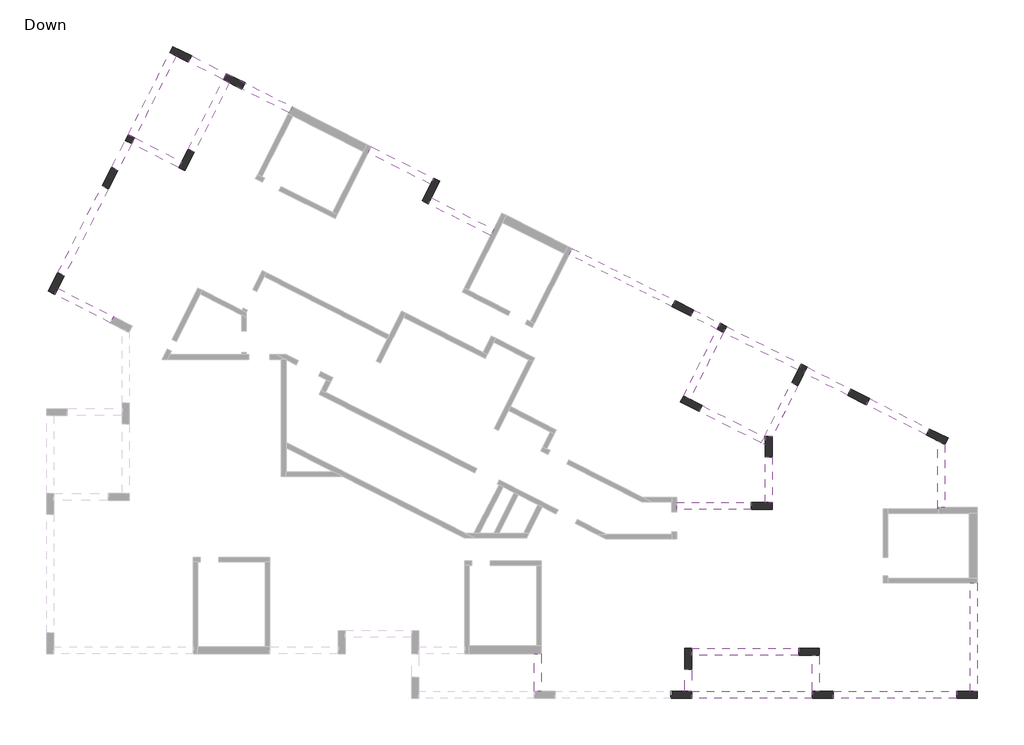
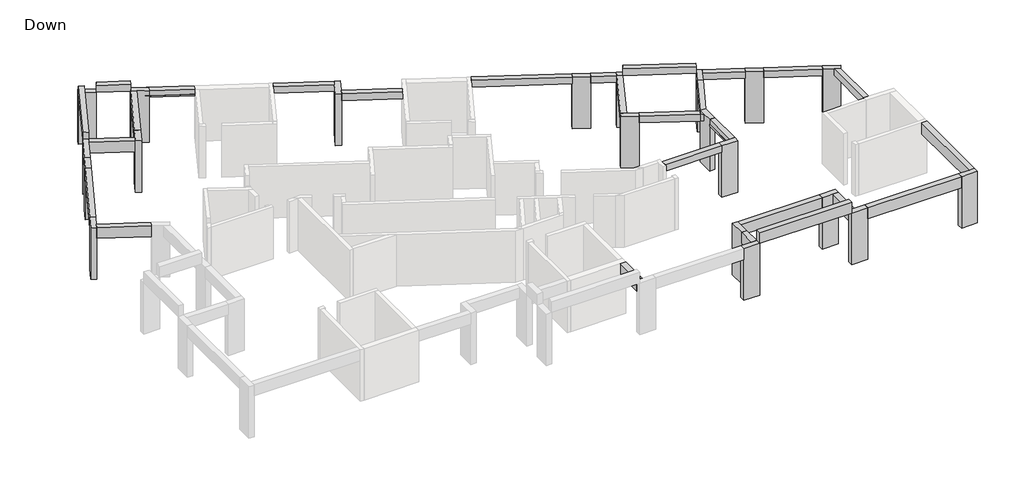
# One storey, part 3 of 3: 28 beams, 20 columns.
"""IFC4 building model written with IfcOpenShell, lengths in millimetres."""

import ifcopenshell
import ifcopenshell.guid

model = None  # the IFC model being written
_history = None  # IfcOwnerHistory: only IFC2X3 demands one
_inside = {}  # id of a spatial element -> (the spatial element, [elements in it])
_under = {}  # id of a project, library or spatial element -> (it, [spatial elements below it])
_declared = {}  # id of a project -> (the project, [libraries it declares])
_typed = {}  # id of a type object -> (the type object, [elements of that type])
_made_of = {}  # id of a material, layer set ... -> (it, [elements and type objects made of it])


def new_model(schema):
    """Start an empty IFC model of exactly this schema.

    Asked for "IFC4X3", IfcOpenShell would pick the latest addendum, in which some entities
    have other attributes; the version numbers below select the first issue.
    IFC2X3 requires an IfcOwnerHistory on every rooted entity: one is made here for all.
    """
    global model, _history
    if schema == "IFC4X3":
        model = ifcopenshell.file(schema_version=(4, 3, 0, 0))
    else:
        model = ifcopenshell.file(schema=schema)
    _inside.clear()
    _under.clear()
    _declared.clear()
    _typed.clear()
    _made_of.clear()
    _history = None
    if model.schema == "IFC2X3":
        org = make("IfcOrganization", Name="unknown")
        user = make(
            "IfcPersonAndOrganization",
            ThePerson=make("IfcPerson", FamilyName="unknown"),
            TheOrganization=org,
        )
        app = make(
            "IfcApplication",
            ApplicationDeveloper=org,
            Version="unknown",
            ApplicationFullName="unknown",
            ApplicationIdentifier="unknown",
        )
        _history = make(
            "IfcOwnerHistory",
            OwningUser=user,
            OwningApplication=app,
            ChangeAction="ADDED",
            CreationDate=0,
        )
    return model


def make(cls, **values):
    """One entity of the class cls with the attributes given. An attribute that is None is left unset."""
    return model.create_entity(
        cls, **{name: value for name, value in values.items() if value is not None}
    )


def rooted(cls, **values):
    """An entity with a GlobalId (a new one), such as an element, a storey or a relation."""
    return make(cls, GlobalId=ifcopenshell.guid.new(), OwnerHistory=_history, **values)


def si_unit(unit_type, name, prefix=None):
    """IfcSIUnit, for example si_unit("LENGTHUNIT", "METRE", prefix="MILLI")."""
    return make("IfcSIUnit", UnitType=unit_type, Prefix=prefix, Name=name)


def assignment(units):
    """IfcUnitAssignment: the units of a project."""
    return None if units is None else make("IfcUnitAssignment", Units=units)


def point(xyz):
    """IfcCartesianPoint."""
    return None if xyz is None else make("IfcCartesianPoint", Coordinates=xyz)


def direction(xyz):
    """IfcDirection."""
    return None if xyz is None else make("IfcDirection", DirectionRatios=xyz)


def frame(location, z_axis=None, x_axis=None):
    """IfcAxis2Placement3D, a coordinate frame: its origin and axes. An axis left out is left unset."""
    return make(
        "IfcAxis2Placement3D",
        Location=point(location),
        Axis=direction(z_axis),
        RefDirection=direction(x_axis),
    )


def origin():
    """The frame at (0, 0, 0) with its axes left unset."""
    return frame((0.0, 0.0, 0.0))


def origin_with_axes():
    """The frame at (0, 0, 0) with the z axis (0, 0, 1) and the x axis (1, 0, 0) written out."""
    return frame((0.0, 0.0, 0.0), z_axis=(0.0, 0.0, 1.0), x_axis=(1.0, 0.0, 0.0))


def place(relative_to, where):
    """IfcLocalPlacement: puts the frame where relative to a parent placement (None: the world)."""
    return make(
        "IfcLocalPlacement", PlacementRelTo=relative_to, RelativePlacement=where
    )


def context(
    kind, dimensions, precision=None, world=None, true_north=None, identifier=None
):
    """IfcGeometricRepresentationContext, for example the 3D "Model" context."""
    return make(
        "IfcGeometricRepresentationContext",
        ContextIdentifier=identifier,
        ContextType=kind,
        CoordinateSpaceDimension=dimensions,
        Precision=precision,
        WorldCoordinateSystem=world,
        TrueNorth=true_north,
    )


def project(units=None, contexts=None):
    """IfcProject with its units and contexts."""
    return rooted(
        "IfcProject",
        Name="project",
        RepresentationContexts=contexts,
        UnitsInContext=assignment(units),
    )


def spatial(cls, under=None, at=None, **own):
    """A site, building, storey or space (cls), placed at a placement, below another one or the project."""
    s = rooted(cls, ObjectPlacement=at, **own)
    if under is not None:
        _under.setdefault(under.id(), (under, []))[1].append(s)
    return s


def polyline(points):
    """IfcPolyline through the points."""
    return make("IfcPolyline", Points=[point(p) for p in points])


def outline(outer, holes=None, kind="AREA"):
    """IfcArbitraryClosedProfileDef: a profile drawn as a closed curve; with holes, ...WithVoids."""
    if holes is None:
        return make("IfcArbitraryClosedProfileDef", ProfileType=kind, OuterCurve=outer)
    return make(
        "IfcArbitraryProfileDefWithVoids",
        ProfileType=kind,
        OuterCurve=outer,
        InnerCurves=holes,
    )


def extrude(swept, where, along, depth):
    """IfcExtrudedAreaSolid: the profile swept, set in the frame where, extruded along a direction by depth."""
    return make(
        "IfcExtrudedAreaSolid",
        SweptArea=swept,
        Position=where,
        ExtrudedDirection=direction(along),
        Depth=depth,
    )


def faces_of(points, faces, orient=None, outer=None):
    """IfcFace entities. A face is a list of loops; a loop is a list of indices into points, from 0.

    orient and outer hold one flag for each loop. By default every Orientation is true, the
    first loop of a face is its IfcFaceOuterBound and the others are IfcFaceBound.
    """
    made = []
    for i, loops in enumerate(faces):
        bounds = []
        for j, loop in enumerate(loops):
            is_outer = j == 0 if outer is None else outer[i][j]
            bounds.append(
                make(
                    "IfcFaceOuterBound" if is_outer else "IfcFaceBound",
                    Bound=make("IfcPolyLoop", Polygon=[points[k] for k in loop]),
                    Orientation=True if orient is None else orient[i][j],
                )
            )
        made.append(make("IfcFace", Bounds=bounds))
    return made


def faceted_brep(points, faces, orient=None, outer=None, voids=None):
    """IfcFacetedBrep: a solid bounded by flat faces; with voids (closed shells), ...WithVoids."""
    shared = [point(p) for p in points]
    hull = make("IfcClosedShell", CfsFaces=faces_of(shared, faces, orient, outer))
    if voids is None:
        return make("IfcFacetedBrep", Outer=hull)
    return make(
        "IfcFacetedBrepWithVoids",
        Outer=hull,
        Voids=[
            make(cls, CfsFaces=faces_of(shared, fs, o, b)) for cls, fs, o, b in voids
        ],
    )


def shape(context_of_items, identifier, shape_type, items):
    """IfcShapeRepresentation: the items that make up one representation, for example the "Body"."""
    return make(
        "IfcShapeRepresentation",
        ContextOfItems=context_of_items,
        RepresentationIdentifier=identifier,
        RepresentationType=shape_type,
        Items=items,
    )


def made_of(thing, what):
    """Note that an element or type object is made of a material, layer set ...; save() writes the relation."""
    if what is not None:
        _made_of.setdefault(what.id(), (what, []))[1].append(thing)
    return thing


def element(
    cls,
    number,
    at=None,
    inside=None,
    cuts=None,
    type_object=None,
    material=None,
    context=None,
    identifier="Body",
    shape_type=None,
    held_by="IfcProductDefinitionShape",
    body=None,
    shapes=None,
    **own,
):
    """One element of the class cls, such as IfcWall. Its Tag is "e" and its number.

    at: its placement. inside: the storey or other place that contains it. cuts: it is an
    opening in that element (IfcRelVoidsElement). A single representation is given by context,
    identifier, shape_type and body (its items); several are given by shapes. held_by: the class
    of the entity that holds the representations. save() writes the other relations.
    """
    e = rooted(cls, Tag="e%d" % number, ObjectPlacement=at, **own)
    if body is not None:
        shapes = [shape(context, identifier, shape_type, body)]
    if shapes is not None:
        e.Representation = make(held_by, Representations=shapes)
    if inside is not None:
        _inside.setdefault(inside.id(), (inside, []))[1].append(e)
    if cuts is not None:
        rooted(
            "IfcRelVoidsElement", RelatingBuildingElement=cuts, RelatedOpeningElement=e
        )
    if type_object is not None:
        _typed.setdefault(type_object.id(), (type_object, []))[1].append(e)
    return made_of(e, material)


def aggregate(whole, parts):
    """IfcRelAggregates: a whole, such as a stair, and the parts it consists of."""
    return rooted("IfcRelAggregates", RelatingObject=whole, RelatedObjects=parts)


def save(model, path):
    """Write the relations noted so far, then the file.

    IfcRelAggregates (storeys below a building ...), IfcRelContainedInSpatialStructure (elements
    in a storey), IfcRelDefinesByType, IfcRelAssociatesMaterial and IfcRelDeclares: one each for
    every whole, place, type object, material and project.
    """
    for whole, parts in _under.values():
        aggregate(whole, parts)
    for where, things in _inside.values():
        rooted(
            "IfcRelContainedInSpatialStructure",
            RelatedElements=things,
            RelatingStructure=where,
        )
    for kind, things in _typed.values():
        rooted("IfcRelDefinesByType", RelatedObjects=things, RelatingType=kind)
    for what, things in _made_of.values():
        rooted("IfcRelAssociatesMaterial", RelatedObjects=things, RelatingMaterial=what)
    for by, libraries in _declared.values():
        rooted("IfcRelDeclares", RelatingContext=by, RelatedDefinitions=libraries)
    model.write(path)


model = new_model("IFC4")

# Units and contexts
model_context = context("Model", 3, world=origin())
ifc_project = project(units=[si_unit("LENGTHUNIT", "METRE", prefix="MILLI")], contexts=[model_context])

# Site, building, storey
site = spatial("IfcSite", under=ifc_project)
building = spatial("IfcBuilding", under=site)
storey = spatial("IfcBuildingStorey", under=building, Name="Down", Elevation=0.0)

# Beams
placement = place(None, origin())
element("IfcBeam", 1, ObjectType="Concrete Rectengular Beam : 30/40", at=placement, inside=storey, context=model_context, shape_type="Brep", body=[
    faceted_brep([(18324.1024442, -5390.1200149, 3080.0), (18322.3676733, -5393.5542971, 3080.0), (18024.1024442, -5242.8905469, 3080.0), (18024.1024442, -8167.1461487, 3080.0), (18025.5784419, -8167.1461487, 3080.0), (18025.5784419, -8117.1461487, 3080.0), (18324.1024442, -8117.1461487, 3080.0), (18324.1024442, -5390.1200149, 2680.0), (18324.1024442, -8117.1461487, 2680.0), (18322.3676733, -5393.5542971, 2680.0), (18025.5784419, -8117.1461487, 2680.0), (18025.5784419, -8167.1461487, 2680.0), (18024.1024442, -8167.1461487, 2680.0), (18024.1024442, -5242.8905469, 2680.0), (18024.1024442, -5242.8905469, 2780.0), (18024.1024442, -8167.1461487, 2780.0)], [[[0, 1, 2, 3, 4, 5, 6]], [[7, 0, 6, 8]], [[9, 7, 8, 10, 11, 12, 13]], [[3, 2, 14, 13, 12, 15]], [[9, 1, 0, 7]], [[1, 9, 13, 14, 2]], [[5, 10, 8, 6]], [[10, 5, 4, 11]], [[4, 3, 15, 12, 11]]]),
])
element("IfcBeam", 2, ObjectType="Concrete Rectengular Beam : 30/40", at=placement, inside=storey, context=model_context, shape_type="Brep", body=[
    faceted_brep([(15078.2317571, -3418.7309173, 3080.0), (14942.9691088, -3686.5069729, 3080.0), (17519.0395063, -4987.7663524, 3080.0), (17654.3021546, -4719.9902967, 3080.0), (15078.2317571, -3418.7309173, 2680.0), (17654.3021546, -4719.9902967, 2680.0), (14942.9691088, -3686.5069729, 2680.0), (17519.0395063, -4987.7663524, 2680.0), (14942.9691088, -3686.5069729, 2780.0), (17519.0395063, -4987.7663524, 2780.0)], [[[0, 1, 2, 3]], [[4, 0, 3, 5]], [[6, 4, 5, 7]], [[2, 1, 8, 6, 7, 9]], [[1, 0, 4, 6, 8]], [[3, 2, 9, 7, 5]]]),
])
element("IfcBeam", 3, ObjectType="Concrete Rectengular Beam : 30/40", at=placement, inside=storey, context=model_context, shape_type="Brep", body=[
    faceted_brep([(14139.6409418, -3280.7190282, 3080.0), (14274.90359, -3012.9429725, 3080.0), (12400.3743588, -2066.0555169, 3080.0), (12265.1117105, -2333.8315725, 3080.0), (14274.90359, -3012.9429725, 2680.0), (12400.3743588, -2066.0555169, 2680.0), (14139.6409418, -3280.7190282, 2680.0), (12265.1117105, -2333.8315725, 2680.0), (12265.1117105, -2333.8315725, 2780.0), (14139.6409418, -3280.7190282, 2780.0)], [[[0, 1, 2, 3]], [[1, 4, 5, 2]], [[4, 6, 7, 5]], [[0, 3, 8, 7, 6, 9]], [[1, 0, 9, 6, 4]], [[3, 2, 5, 7, 8]]]),
])
element("IfcBeam", 4, ObjectType="Concrete Rectengular Beam : 30/40", at=placement, inside=storey, context=model_context, shape_type="Brep", body=[
    faceted_brep([(11994.586414, -2869.3836839, 3080.0), (11726.8103583, -2734.1210356, 3080.0), (10548.8414039, -5066.1164862, 3080.0), (10413.5787556, -5333.8925419, 3080.0), (10583.8347444, -5419.8945403, 3080.0), (10583.8347444, -5041.560553, 3080.0), (10883.8347444, -5041.560553, 3080.0), (10883.8347444, -5068.3107696, 3080.0), (11726.8103583, -2734.1210356, 2680.0), (10548.8414039, -5066.1164862, 2680.0), (10413.5787556, -5333.8925419, 2680.0), (10413.5787556, -5333.8925419, 2780.0), (11994.586414, -2869.3836839, 2680.0), (10883.8347444, -5068.3107696, 2680.0), (10883.8347444, -5041.560553, 2680.0), (10583.8347444, -5041.560553, 2680.0), (10583.8347444, -5419.8945403, 2680.0), (10883.8347444, -5068.3107696, 2780.0), (11994.586414, -2869.3836839, 2780.0), (10583.8347444, -5419.8945403, 2780.0)], [[[0, 1, 2, 3, 4, 5, 6, 7]], [[1, 8, 9, 10, 11, 3, 2]], [[8, 12, 13, 14, 15, 16, 10, 9]], [[0, 7, 17, 13, 12, 18]], [[1, 0, 18, 12, 8]], [[6, 14, 13, 17, 7]], [[15, 5, 4, 19, 16]], [[5, 15, 14, 6]], [[4, 3, 11, 10, 16, 19]]]),
])
element("IfcBeam", 5, ObjectType="Concrete Rectengular Beam : 30/40", at=placement, inside=storey, context=model_context, shape_type="Brep", body=[
    faceted_brep([(7870.7444656, -3713.3200862, 3080.0), (7735.4818174, -3981.0961419, 3080.0), (10413.5787556, -5333.8925419, 3080.0), (10548.8414039, -5066.1164862, 3080.0), (7870.7444656, -3713.3200862, 2680.0), (10548.8414039, -5066.1164862, 2680.0), (7735.4818174, -3981.0961419, 2680.0), (10413.5787556, -5333.8925419, 2680.0), (7735.4818174, -3981.0961419, 2780.0), (10413.5787556, -5333.8925419, 2780.0)], [[[0, 1, 2, 3]], [[4, 0, 3, 5]], [[6, 4, 5, 7]], [[2, 1, 8, 6, 7, 9]], [[1, 0, 4, 6, 8]], [[3, 2, 9, 7, 5]]]),
])
element("IfcBeam", 6, ObjectType="Concrete Rectengular Beam : 30/40", at=placement, inside=storey, context=model_context, shape_type="Brep", body=[
    faceted_brep([(7335.1923543, -3442.7947897, 3080.0), (8783.6866053, -575.2472278, 3080.0), (8515.9105496, -439.9845796, 3080.0), (7067.4162986, -3307.5321414, 3080.0), (8515.9105496, -439.9845796, 2780.0), (8515.9105496, -439.9845796, 2680.0), (7067.4162986, -3307.5321414, 2680.0), (7067.4162986, -3307.5321414, 2780.0), (8783.6866053, -575.2472278, 2680.0), (7335.1923543, -3442.7947897, 2680.0)], [[[0, 1, 2, 3]], [[3, 2, 4, 5, 6, 7]], [[6, 5, 8, 9]], [[1, 0, 9, 8]], [[0, 3, 7, 6, 9]], [[1, 8, 5, 4, 2]]]),
])
element("IfcBeam", 7, ObjectType="Concrete Rectengular Beam : 30/40", at=placement, inside=storey, context=model_context, shape_type="Brep", body=[
    faceted_brep([(7509.3028963, 404.5883841, 3080.0), (7374.040248, 136.8123284, 3080.0), (8515.9105496, -439.9845796, 3080.0), (8651.1731978, -172.2085239, 3080.0), (8651.1731978, -172.2085239, 2680.0), (7509.3028963, 404.5883841, 2680.0), (7374.040248, 136.8123284, 2680.0), (8515.9105496, -439.9845796, 2680.0), (7374.040248, 136.8123284, 2780.0), (8515.9105496, -439.9845796, 2780.0)], [[[0, 1, 2, 3]], [[3, 4, 5, 0]], [[6, 5, 4, 7]], [[2, 1, 8, 6, 7, 9]], [[1, 0, 5, 6, 8]], [[3, 2, 9, 7, 4]]]),
])
element("IfcBeam", 8, ObjectType="Concrete Rectengular Beam : 30/40", at=placement, inside=storey, context=model_context, shape_type="Brep", body=[
    faceted_brep([(6570.712081, 542.6002731, 3080.0), (6705.9747293, 810.3763288, 3080.0), (2279.1613083, 3046.5079542, 3080.0), (2143.8361829, 2778.7634578, 3080.0), (6705.9747293, 810.3763288, 2680.0), (2279.1613083, 3046.5079542, 2680.0), (6570.712081, 542.6002731, 2680.0), (2143.8361829, 2778.7634578, 2680.0), (2143.8361829, 2778.7634578, 2780.0), (6570.712081, 542.6002731, 2780.0)], [[[0, 1, 2, 3]], [[1, 4, 5, 2]], [[4, 6, 7, 5]], [[0, 3, 8, 7, 6, 9]], [[1, 0, 9, 6, 4]], [[3, 2, 5, 7, 8]]]),
])
element("IfcBeam", 9, ObjectType="Concrete Rectengular Beam : 30/40", at=placement, inside=storey, context=model_context, shape_type="Brep", body=[
    faceted_brep([(-3788.4112388, 5231.6305271, 3080.0), (-3923.6738871, 4963.8544714, 3080.0), (-1236.2326264, 3606.3379414, 3080.0), (-1101.4629559, 3874.3630166, 3080.0), (-3923.6738871, 4963.8544714, 2780.0), (-3923.6738871, 4963.8544714, 2680.0), (-1236.2326264, 3606.3379414, 2680.0), (-1236.2326264, 3606.3379414, 2780.0), (-3788.4112388, 5231.6305271, 2680.0), (-1101.4629559, 3874.3630166, 2680.0)], [[[0, 1, 2, 3]], [[2, 1, 4, 5, 6, 7]], [[5, 8, 9, 6]], [[8, 0, 3, 9]], [[1, 0, 8, 5, 4]], [[3, 2, 7, 6, 9]]]),
])
element("IfcBeam", 10, ObjectType="Concrete Rectengular Beam : 30/40", at=placement, inside=storey, context=model_context, shape_type="Brep", body=[
    faceted_brep([(-3695.4868992, 6080.9626571, 3080.0), (-3830.7495474, 5813.1866015, 3080.0), (-3830.7495474, 5813.1866015, 2780.0), (-3830.7495474, 5813.1866015, 2680.0), (-3695.4868992, 6080.9626571, 2680.0), (-6512.212519, 7167.6832976, 3080.0), (-6377.2019242, 7435.5866739, 3080.0), (-6377.2019242, 7435.5866739, 2680.0), (-6512.212519, 7167.6832976, 2680.0), (-6512.212519, 7167.6832976, 2780.0)], [[[0, 1, 2, 3, 4]], [[5, 6, 7, 8, 9]], [[1, 5, 9, 8, 3, 2]], [[1, 0, 6, 5]], [[7, 6, 0, 4]], [[4, 3, 8, 7]]]),
])
element("IfcBeam", 11, ObjectType="Concrete Rectengular Beam : 30/40", at=placement, inside=storey, context=model_context, shape_type="Brep", body=[
    faceted_brep([(-12614.1088599, 10586.0571178, 3080.0), (-12749.6797072, 10318.4367438, 3080.0), (-12481.9034742, 10183.1740059, 3080.0), (-12479.6439601, 10187.6343455, 3080.0), (-11943.8088624, 9916.9661031, 3080.0), (-9919.3091434, 8894.3235346, 3080.0), (-9785.6009014, 9157.2830771, 3080.0), (-12614.1088599, 10586.0571178, 2680.0), (-9785.6009014, 9157.2830771, 2680.0), (-12749.6797072, 10318.4367438, 2680.0), (-9921.5753848, 8889.8665932, 2680.0), (-9921.5753848, 8889.8665932, 2780.0), (-12481.9034742, 10183.1740059, 2780.0), (-9919.3091434, 8894.3235346, 2780.0), (-11943.8088624, 9916.9661031, 2780.0), (-12479.6439601, 10187.6343455, 2780.0)], [[[0, 1, 2, 3, 4, 5, 6]], [[7, 0, 6, 8]], [[9, 7, 8, 10]], [[1, 9, 10, 11, 12, 2]], [[1, 0, 7, 9]], [[10, 8, 6, 5, 13, 11]], [[13, 14, 15, 12, 11]], [[15, 3, 2, 12]], [[15, 14, 13, 5, 4, 3]]]),
])
element("IfcBeam", 12, ObjectType="Concrete Rectengular Beam : 30/40", at=placement, inside=storey, context=model_context, shape_type="Brep", body=[
    faceted_brep([(10883.8347444, -7886.8724338, 3080.0), (10883.8347444, -5941.560553, 3080.0), (10598.8347444, -5941.560553, 3080.0), (10598.8347444, -7886.8724338, 3080.0), (10583.8347444, -5941.560553, 2680.0), (10583.8347444, -7886.8724338, 2680.0), (10583.8347444, -7886.8724338, 2780.0), (10583.8347444, -5941.560553, 2780.0), (10883.8347444, -5941.560553, 2680.0), (10883.8347444, -7886.8724338, 2680.0), (10883.8347444, -7886.8724338, 2780.0), (10883.8347444, -5941.560553, 2780.0), (10598.8347444, -5941.560553, 2780.0), (10598.8347444, -7886.8724338, 2780.0)], [[[0, 1, 2, 3]], [[4, 5, 6, 7]], [[4, 8, 9, 5]], [[1, 0, 10, 9, 8, 11]], [[8, 4, 7, 12, 2, 1, 11]], [[5, 9, 10, 0, 3, 13, 6]], [[13, 12, 7, 6]], [[12, 13, 3, 2]]]),
])
element("IfcBeam", 13, ObjectType="Concrete Rectengular Beam : 30/40", at=placement, inside=storey, context=model_context, shape_type="Brep", body=[
    faceted_brep([(9983.8347444, -8186.8724338, 3080.0), (9983.8347444, -7886.8724338, 3080.0), (6770.8726693, -7886.8724338, 3080.0), (6770.8726693, -8186.8724338, 3080.0), (9983.8347444, -7886.8724338, 2680.0), (6770.8726693, -7886.8724338, 2680.0), (6770.8726693, -7886.8724338, 2780.0), (9983.8347444, -8186.8724338, 2680.0), (6770.8726693, -8186.8724338, 2680.0), (6770.8726693, -8186.8724338, 2780.0), (9983.8347444, -8186.8724338, 2780.0)], [[[0, 1, 2, 3]], [[1, 4, 5, 6, 2]], [[4, 7, 8, 5]], [[0, 3, 9, 8, 7, 10]], [[1, 0, 10, 7, 4]], [[3, 2, 6, 5, 8, 9]]]),
])
element("IfcBeam", 14, ObjectType="Concrete Rectengular Beam : 30/40", at=placement, inside=storey, context=model_context, shape_type="SweptSolid", body=[
    extrude(outline(polyline([(8783.6866053, -575.2472278), (8918.9492535, -307.4711721), (12131.2236827, -1930.0985019), (11995.9610344, -2197.8745575), (8783.6866053, -575.2472278)])), frame((0.0, 0.0, 3080.0), z_axis=(0.0, 0.0, 1.0), x_axis=(1.0, 0.0, 0.0)), (0.0, 0.0, 1.0), 400.0),
])
element("IfcBeam", 15, ObjectType="Concrete Rectengular Beam : 30/40", at=placement, inside=storey, context=model_context, shape_type="SweptSolid", body=[
    extrude(outline(polyline([(-14249.2038057, 11075.8965553), (-14113.9411575, 11343.672611), (-12614.2787114, 10586.1429155), (-12749.5413596, 10318.3668598), (-14249.2038057, 11075.8965553)])), frame((0.0, 0.0, 3080.0), z_axis=(0.0, 0.0, 1.0), x_axis=(1.0, 0.0, 0.0)), (0.0, 0.0, 1.0), 400.0),
])
element("IfcBeam", 16, ObjectType="Concrete Rectengular Beam : 30/40", at=placement, inside=storey, context=model_context, shape_type="SweptSolid", body=[
    extrude(outline(polyline([(-16564.6681031, 7822.7745567), (-16832.4441588, 7958.0372049), (-15052.5319727, 11481.6845001), (-14784.755917, 11346.4218518), (-16564.6681031, 7822.7745567)])), frame((0.0, 0.0, 3080.0), z_axis=(0.0, 0.0, 1.0), x_axis=(1.0, 0.0, 0.0)), (0.0, 0.0, 1.0), 400.0),
])
element("IfcBeam", 17, ObjectType="Concrete Rectengular Beam : 30/65", at=placement, inside=storey, context=model_context, shape_type="Brep", body=[
    faceted_brep([(-17475.2288855, 111.6100244, 3080.0), (-19872.740079, 1333.8706328, 3080.0), (-20008.9963132, 1066.5987888, 3080.0), (-17611.4851198, -155.6618196, 3080.0), (-17475.2288855, 111.6100244, 2780.0), (-17475.2288855, 111.6100244, 2430.0), (-19872.740079, 1333.8706328, 2430.0), (-19872.740079, 1333.8706328, 2780.0), (-17611.4851198, -155.6618196, 2430.0), (-20008.9963132, 1066.5987888, 2430.0)], [[[0, 1, 2, 3]], [[1, 0, 4, 5, 6, 7]], [[6, 5, 8, 9]], [[2, 9, 8, 3]], [[2, 1, 7, 6, 9]], [[3, 8, 5, 4, 0]]]),
])
element("IfcBeam", 18, ObjectType="Concrete Rectengular Beam : 30/65", at=placement, inside=storey, context=model_context, shape_type="Brep", body=[
    faceted_brep([(-17692.9134653, 5609.6843751, 3080.0), (-17960.1853094, 5745.9406093, 3080.0), (-19867.4994546, 2004.6705552, 3080.0), (-19600.2276105, 1868.414321, 3080.0), (-19600.2276105, 1868.414321, 2780.0), (-19600.2276105, 1868.414321, 2430.0), (-17692.9134653, 5609.6843751, 2430.0), (-17692.9134653, 5609.6843751, 2780.0), (-17960.1853094, 5745.9406093, 2430.0), (-19867.4994546, 2004.6705552, 2430.0)], [[[0, 1, 2, 3]], [[0, 3, 4, 5, 6, 7]], [[8, 6, 5, 9]], [[1, 8, 9, 2]], [[1, 0, 7, 6, 8]], [[2, 9, 5, 4, 3]]]),
])
element("IfcBeam", 19, ObjectType="Concrete Rectengular Beam : 30/65", at=placement, inside=storey, context=model_context, shape_type="Brep", body=[
    faceted_brep([(-17551.4166067, 6547.7561415, 3080.0), (-17284.1447626, 6411.4999073, 3080.0), (-16701.0058274, 7555.3493571, 3080.0), (-16564.7491456, 7822.622079, 3080.0), (-16832.3702214, 7958.1932819, 3080.0), (-16564.7491456, 7822.622079, 2430.0), (-17284.1447626, 6411.4999073, 2780.0), (-17284.1447626, 6411.4999073, 2430.0), (-16701.0058274, 7555.3493571, 2430.0), (-17551.4166067, 6547.7561415, 2430.0), (-16832.3702214, 7958.1932819, 2430.0)], [[[0, 1, 2, 3, 4]], [[5, 3, 2, 1, 6, 7, 8]], [[7, 9, 10, 5, 8]], [[9, 0, 4, 10]], [[1, 0, 9, 7, 6]], [[4, 3, 5, 10]]]),
])
element("IfcBeam", 20, ObjectType="Concrete Rectengular Beam : 30/65", at=placement, inside=storey, context=model_context, shape_type="Brep", body=[
    faceted_brep([(-16564.7491456, 7822.622079, 3080.0), (-16701.0058274, 7555.3493571, 3080.0), (-14671.1406915, 6527.0624132, 3080.0), (-14535.569934, 6794.6826099, 3080.0), (-16701.0058274, 7555.3493571, 2780.0), (-16701.0058274, 7555.3493571, 2430.0), (-14671.1406915, 6527.0624132, 2430.0), (-14671.1406915, 6527.0624132, 2780.0), (-16564.7491456, 7822.622079, 2430.0), (-14535.569934, 6794.6826099, 2430.0)], [[[0, 1, 2, 3]], [[2, 1, 4, 5, 6, 7]], [[5, 8, 9, 6]], [[8, 0, 3, 9]], [[1, 0, 8, 5, 4]], [[3, 2, 7, 6, 9]]]),
])
element("IfcBeam", 21, ObjectType="Concrete Rectengular Beam : 30/65", at=placement, inside=storey, context=model_context, shape_type="Brep", body=[
    faceted_brep([(-12749.6795392, 10318.4370754, 2430.0), (-12749.6795392, 10318.4370754, 3080.0), (-12749.3914068, 10318.2911136, 3080.0), (-12482.0593425, 10182.8663179, 3080.0), (-12482.0593425, 10182.8663179, 2780.0), (-12482.0593425, 10182.8663179, 2430.0), (-12749.3914068, 10318.2911136, 2430.0), (-14263.767467, 7329.5881791, 3080.0), (-13996.1472702, 7194.0174215, 3080.0), (-13996.1472702, 7194.0174215, 2780.0), (-13996.1472702, 7194.0174215, 2430.0), (-14263.767467, 7329.5881791, 2430.0)], [[[0, 1, 2, 3, 4, 5, 6]], [[7, 8, 3, 2, 1]], [[3, 8, 9, 10, 5, 4]], [[10, 11, 0, 6, 5]], [[1, 0, 11, 7]], [[8, 7, 11, 10, 9]]]),
])
element("IfcBeam", 22, ObjectType="Concrete Rectengular Beam : 30/65", at=placement, inside=storey, context=model_context, shape_type="Brep", body=[
    faceted_brep([(645.0940817, -16035.9823018, 3080.0), (945.0940817, -16035.9823018, 3080.0), (945.0940817, -14416.2328988, 3080.0), (645.0940817, -14416.2328988, 3080.0), (645.0940817, -16035.9823018, 2430.0), (645.0940817, -14416.2328988, 2430.0), (945.0940817, -16035.9823018, 2430.0), (945.0940817, -14416.2328988, 2430.0), (945.0940817, -16035.9823018, 2780.0)], [[[0, 1, 2, 3]], [[4, 0, 3, 5]], [[6, 4, 5, 7]], [[1, 8, 6, 7, 2]], [[1, 0, 4, 6, 8]], [[3, 2, 7, 5]]]),
])
element("IfcBeam", 23, ObjectType="Concrete Rectengular Beam : 30/65", at=placement, inside=storey, context=model_context, shape_type="Brep", body=[
    faceted_brep([(12020.9090644, -14474.4460263, 3080.0), (12020.9090644, -14174.4460263, 3080.0), (7425.6343679, -14174.4460263, 3080.0), (7425.6343679, -14474.4460263, 3080.0), (12020.9090644, -14474.4460263, 2430.0), (7425.6343679, -14474.4460263, 2430.0), (12020.9090644, -14174.4460263, 2430.0), (7425.6343679, -14174.4460263, 2430.0), (12020.9090644, -14174.4460263, 2780.0), (7425.6343679, -14174.4460263, 2780.0)], [[[0, 1, 2, 3]], [[4, 0, 3, 5]], [[6, 4, 5, 7]], [[2, 1, 8, 6, 7, 9]], [[1, 0, 4, 6, 8]], [[3, 2, 9, 7, 5]]]),
])
element("IfcBeam", 24, ObjectType="Concrete Rectengular Beam : 30/65", at=placement, inside=storey, context=model_context, shape_type="Brep", body=[
    faceted_brep([(12620.9090644, -16035.9823018, 3080.0), (12920.9090644, -16035.9823018, 3080.0), (12920.9090644, -14474.4460263, 3080.0), (12620.9090644, -14474.4460263, 3080.0), (12920.9090644, -16035.9823018, 2780.0), (12920.9090644, -16035.9823018, 2430.0), (12920.9090644, -14474.4460263, 2430.0), (12920.9090644, -14474.4460263, 2780.0), (12620.9090644, -16035.9823018, 2430.0), (12620.9090644, -14474.4460263, 2430.0)], [[[0, 1, 2, 3]], [[2, 1, 4, 5, 6, 7]], [[5, 8, 9, 6]], [[8, 0, 3, 9]], [[1, 0, 8, 5, 4]], [[3, 2, 7, 6, 9]]]),
])
element("IfcBeam", 25, ObjectType="Concrete Rectengular Beam : 30/65", at=placement, inside=storey, context=model_context, shape_type="SweptSolid", body=[
    extrude(outline(polyline([(13520.9090644, -16335.9823018), (13520.9090644, -16035.9823018), (18824.1024442, -16035.9823018), (18824.1024442, -16335.9823018), (13520.9090644, -16335.9823018)])), frame((0.0, 0.0, 2430.0), z_axis=(0.0, 0.0, 1.0), x_axis=(1.0, 0.0, 0.0)), (0.0, 0.0, 1.0), 650.0),
])
element("IfcBeam", 26, ObjectType="Concrete Rectengular Beam : 30/65", at=placement, inside=storey, context=model_context, shape_type="Brep", body=[
    faceted_brep([(19724.1024442, -11368.4141282, 3080.0), (19424.1024442, -11368.4141282, 3080.0), (19424.1024442, -16035.9823018, 3080.0), (19724.1024442, -16035.9823018, 3080.0), (19724.1024442, -11368.4141282, 2430.0), (19724.1024442, -16035.9823018, 2430.0), (19424.1024442, -11368.4141282, 2430.0), (19424.1024442, -16035.9823018, 2430.0), (19424.1024442, -11368.4141282, 2780.0), (19424.1024442, -16035.9823018, 2780.0)], [[[0, 1, 2, 3]], [[4, 0, 3, 5]], [[6, 4, 5, 7]], [[1, 8, 6, 7, 9, 2]], [[1, 0, 4, 6, 8]], [[3, 2, 9, 7, 5]]]),
])
element("IfcBeam", 27, ObjectType="Concrete Rectengular Beam : 30/65", at=placement, inside=storey, context=model_context, shape_type="Brep", body=[
    faceted_brep([(7125.6343679, -16035.9823018, 3080.0), (7425.6343679, -16035.9823018, 3080.0), (7425.6343679, -15074.4460263, 3080.0), (7125.6343679, -15074.4460263, 3080.0), (7125.6343679, -15074.4460263, 2780.0), (7125.6343679, -15074.4460263, 2430.0), (7125.6343679, -16035.9823018, 2430.0), (7125.6343679, -16035.9823018, 2780.0), (7425.6343679, -16035.9823018, 2430.0), (7425.6343679, -15074.4460263, 2430.0)], [[[0, 1, 2, 3]], [[0, 3, 4, 5, 6, 7]], [[8, 6, 5, 9]], [[1, 8, 9, 2]], [[1, 0, 7, 6, 8]], [[3, 2, 9, 5, 4]]]),
])
element("IfcBeam", 28, ObjectType="Concrete Rectengular Beam : 30/65", at=placement, inside=storey, context=model_context, shape_type="SweptSolid", body=[
    extrude(outline(polyline([(12620.9090644, -16035.9823018), (12620.9090644, -16335.9823018), (7425.6343679, -16335.9823018), (7425.6343679, -16035.9823018), (12620.9090644, -16035.9823018)])), frame((0.0, 0.0, 3080.0), z_axis=(0.0, 0.0, 1.0), x_axis=(1.0, 0.0, 0.0)), (0.0, 0.0, 1.0), 650.0),
])

# Columns
element("IfcColumn", 29, ObjectType="Concrete Rectengular Column : 30/110", at=placement, inside=storey, context=model_context, shape_type="Brep", body=[
    faceted_brep([(-4191.4499427, 5099.1171197, 0.0), (-3695.4868992, 6080.9626571, 0.0), (-3427.7108435, 5945.7000089, 0.0), (-3923.6738871, 4963.8544714, 0.0), (-4191.4499427, 5099.1171197, 3080.0), (-3830.7495474, 5813.1866015, 3080.0), (-3695.4868992, 6080.9626571, 3080.0), (-4191.4499427, 5099.1171197, 2780.0), (-3427.7108435, 5945.7000089, 3080.0), (-3923.6738871, 4963.8544714, 3080.0)], [[[0, 1, 2, 3]], [[4, 5, 6, 1, 0, 7]], [[6, 8, 2, 1]], [[8, 9, 3, 2]], [[9, 4, 7, 0, 3]], [[4, 9, 8, 6, 5]]]),
])
element("IfcColumn", 30, ObjectType="Concrete Rectengular Column : 30/30", at=placement, inside=storey, context=model_context, shape_type="Brep", body=[
    faceted_brep([(-16564.74248, 7822.6187024, 0.0), (-16700.3132376, 7554.9985056, 0.0), (-16967.9334343, 7690.5692632, 0.0), (-16832.3626767, 7958.1894599, 0.0), (-16564.74248, 7822.6187024, 3080.0), (-16700.3132376, 7554.9985056, 3080.0), (-16701.0058274, 7555.3493571, 3080.0), (-16967.9334343, 7690.5692632, 3080.0), (-16832.3626767, 7958.1894599, 3080.0)], [[[0, 1, 2, 3]], [[4, 5, 1, 0]], [[5, 6, 7, 2, 1]], [[7, 8, 3, 2]], [[8, 4, 0, 3]], [[4, 8, 7, 6, 5]]]),
])
element("IfcColumn", 31, ObjectType="Concrete Rectengular Column : 30/30", at=placement, inside=storey, context=model_context, shape_type="Brep", body=[
    faceted_brep([(8651.1731978, -172.2085239, 0.0), (8918.9492535, -307.4711721, 0.0), (8783.6866053, -575.2472278, 0.0), (8515.9105496, -439.9845796, 0.0), (8651.1731978, -172.2085239, 3080.0), (8918.9492535, -307.4711721, 3080.0), (8783.6866053, -575.2472278, 3080.0), (8783.6866053, -575.2472278, 2680.0), (8515.9105496, -439.9845796, 3080.0), (8515.9105496, -439.9845796, 2680.0)], [[[0, 1, 2, 3]], [[4, 5, 1, 0]], [[5, 6, 7, 2, 1]], [[6, 8, 9, 3, 2, 7]], [[8, 4, 0, 3, 9]], [[4, 8, 6, 5]]]),
])
element("IfcColumn", 32, ObjectType="Concrete Rectengular Column : 30/90", at=placement, inside=storey, context=model_context, shape_type="Brep", body=[
    faceted_brep([(6525.6343679, -16035.9823018, 0.0), (7425.6343679, -16035.9823018, 0.0), (7425.6343679, -16335.9823018, 0.0), (6525.6343679, -16335.9823018, 0.0), (6525.6343679, -16035.9823018, 3080.0), (7125.6343679, -16035.9823018, 3080.0), (7425.6343679, -16035.9823018, 3080.0), (7425.6343679, -16335.9823018, 3080.0), (6525.6343679, -16335.9823018, 3080.0)], [[[0, 1, 2, 3]], [[4, 5, 6, 1, 0]], [[6, 7, 2, 1]], [[7, 8, 3, 2]], [[8, 4, 0, 3]], [[4, 8, 7, 6, 5]]]),
])
element("IfcColumn", 33, ObjectType="Concrete Rectengular Column : 30/90", at=placement, inside=storey, context=model_context, shape_type="Brep", body=[
    faceted_brep([(7125.6343679, -15074.4460263, 0.0), (7125.6343679, -14174.4460263, 0.0), (7425.6343679, -14174.4460263, 0.0), (7425.6343679, -15074.4460263, 0.0), (7125.6343679, -15074.4460263, 3080.0), (7125.6343679, -14174.4460263, 3080.0), (7125.6343679, -14174.4460263, 2780.0), (7425.6343679, -14174.4460263, 3080.0), (7425.6343679, -15074.4460263, 3080.0)], [[[0, 1, 2, 3]], [[4, 5, 6, 1, 0]], [[5, 7, 2, 1, 6]], [[7, 8, 3, 2]], [[8, 4, 0, 3]], [[4, 8, 7, 5]]]),
])
element("IfcColumn", 34, ObjectType="Concrete Rectengular Column : 30/90", at=placement, inside=storey, context=model_context, shape_type="Brep", body=[
    faceted_brep([(12920.9090644, -14474.4460263, 0.0), (12020.9090644, -14474.4460263, 0.0), (12020.9090644, -14174.4460263, 0.0), (12920.9090644, -14174.4460263, 0.0), (12920.9090644, -14474.4460263, 3080.0), (12020.9090644, -14474.4460263, 3080.0), (12020.9090644, -14174.4460263, 3080.0), (12920.9090644, -14174.4460263, 3080.0), (12920.9090644, -14174.4460263, 2780.0)], [[[0, 1, 2, 3]], [[4, 5, 1, 0]], [[5, 6, 2, 1]], [[6, 7, 8, 3, 2]], [[7, 4, 0, 3, 8]], [[4, 7, 6, 5]]]),
])
element("IfcColumn", 35, ObjectType="Concrete Rectengular Column : 30/90", at=placement, inside=storey, context=model_context, shape_type="Brep", body=[
    faceted_brep([(13520.9090644, -16335.9823018, 0.0), (12620.9090644, -16335.9823018, 0.0), (12620.9090644, -16035.9823018, 0.0), (13520.9090644, -16035.9823018, 0.0), (13520.9090644, -16335.9823018, 3080.0), (12620.9090644, -16335.9823018, 3080.0), (12620.9090644, -16035.9823018, 3080.0), (12920.9090644, -16035.9823018, 3080.0), (13520.9090644, -16035.9823018, 3080.0)], [[[0, 1, 2, 3]], [[4, 5, 1, 0]], [[5, 6, 2, 1]], [[6, 7, 8, 3, 2]], [[8, 4, 0, 3]], [[4, 8, 7, 6, 5]]]),
])
element("IfcColumn", 36, ObjectType="Concrete Rectengular Column : 30/90", at=placement, inside=storey, context=model_context, shape_type="Brep", body=[
    faceted_brep([(19724.1024442, -16335.9823018, 0.0), (18824.1024442, -16335.9823018, 0.0), (18824.1024442, -16035.9823018, 0.0), (19724.1024442, -16035.9823018, 0.0), (19724.1024442, -16335.9823018, 3080.0), (18824.1024442, -16335.9823018, 3080.0), (18824.1024442, -16035.9823018, 3080.0), (19424.1024442, -16035.9823018, 3080.0), (19724.1024442, -16035.9823018, 3080.0)], [[[0, 1, 2, 3]], [[4, 5, 1, 0]], [[5, 6, 2, 1]], [[6, 7, 8, 3, 2]], [[8, 4, 0, 3]], [[4, 8, 7, 6, 5]]]),
])
element("IfcColumn", 37, ObjectType="Concrete Rectengular Column : 30/90", at=placement, inside=storey, context=model_context, shape_type="Brep", body=[
    faceted_brep([(17654.3021546, -4719.9902967, 0.0), (18457.6303216, -5125.7782414, 0.0), (18322.3676733, -5393.5542971, 0.0), (17519.0395063, -4987.7663524, 0.0), (17654.3021546, -4719.9902967, 3080.0), (18457.6303216, -5125.7782414, 3080.0), (17654.3021546, -4719.9902967, 2680.0), (18322.3676733, -5393.5542971, 3080.0), (18024.1024442, -5242.8905469, 3080.0), (17519.0395063, -4987.7663524, 3080.0), (17519.0395063, -4987.7663524, 2680.0)], [[[0, 1, 2, 3]], [[4, 5, 1, 0, 6]], [[5, 7, 2, 1]], [[7, 8, 9, 10, 3, 2]], [[9, 4, 6, 0, 3, 10]], [[4, 9, 8, 7, 5]]]),
])
element("IfcColumn", 38, ObjectType="Concrete Rectengular Column : 30/90", at=placement, inside=storey, context=model_context, shape_type="SweptSolid", body=[
    extrude(outline(polyline([(14274.90359, -3012.9429725), (15078.2317571, -3418.7309173), (14942.9691088, -3686.5069729), (14139.6409418, -3280.7190282), (14274.90359, -3012.9429725)])), origin_with_axes(), (0.0, 0.0, 1.0), 3080.0),
])
element("IfcColumn", 39, ObjectType="Concrete Rectengular Column : 30/90", at=placement, inside=storey, context=model_context, shape_type="Brep", body=[
    faceted_brep([(11726.8103583, -2734.1210356, 0.0), (12132.5983031, -1930.7928686, 0.0), (12400.3743588, -2066.0555169, 0.0), (11994.586414, -2869.3836839, 0.0), (11726.8103583, -2734.1210356, 3080.0), (12132.5983031, -1930.7928686, 3080.0), (12400.3743588, -2066.0555169, 3080.0), (12400.3743588, -2066.0555169, 2680.0), (12265.1117105, -2333.8315725, 3080.0), (11994.586414, -2869.3836839, 3080.0)], [[[0, 1, 2, 3]], [[4, 5, 1, 0]], [[5, 6, 7, 2, 1]], [[6, 8, 9, 3, 2, 7]], [[9, 4, 0, 3]], [[4, 9, 8, 6, 5]]]),
])
element("IfcColumn", 40, ObjectType="Concrete Rectengular Column : 30/90", at=placement, inside=storey, context=model_context, shape_type="SweptSolid", body=[
    extrude(outline(polyline([(6705.9747293, 810.3763288), (7509.3028963, 404.5883841), (7374.040248, 136.8123284), (6570.712081, 542.6002731), (6705.9747293, 810.3763288)])), origin_with_axes(), (0.0, 0.0, 1.0), 3080.0),
])
element("IfcColumn", 41, ObjectType="Concrete Rectengular Column : 30/90", at=placement, inside=storey, context=model_context, shape_type="Brep", body=[
    faceted_brep([(-12614.1287586, 10586.0671693, 0.0), (-11810.8005916, 10180.2792245, 0.0), (-11946.0632398, 9912.5031689, 0.0), (-12749.3914069, 10318.2911136, 0.0), (-12614.1287586, 10586.0671693, 3080.0), (-11810.8005916, 10180.2792245, 3080.0), (-11946.0632398, 9912.5031689, 3080.0), (-11946.0632398, 9912.5031689, 2780.0), (-12481.9034742, 10183.1740059, 3080.0), (-12749.3914069, 10318.2911136, 3080.0)], [[[0, 1, 2, 3]], [[4, 5, 1, 0]], [[5, 6, 7, 2, 1]], [[6, 8, 9, 3, 2, 7]], [[9, 4, 0, 3]], [[4, 9, 8, 6, 5]]]),
])
element("IfcColumn", 42, ObjectType="Concrete Rectengular Column : 30/90", at=placement, inside=storey, context=model_context, shape_type="SweptSolid", body=[
    extrude(outline(polyline([(-14917.2693245, 11749.4605557), (-14113.9411575, 11343.672611), (-14249.2038057, 11075.8965553), (-15052.5319727, 11481.6845001), (-14917.2693245, 11749.4605557)])), origin_with_axes(), (0.0, 0.0, 1.0), 3080.0),
])
element("IfcColumn", 43, ObjectType="Concrete Rectengular Column : 30/90", at=placement, inside=storey, context=model_context, shape_type="Brep", body=[
    faceted_brep([(-14670.4797396, 6526.7275889, 0.0), (-14263.767467, 7329.5881791, 0.0), (-13996.1472702, 7194.0174215, 0.0), (-14402.8595429, 6391.1568314, 0.0), (-14670.4797396, 6526.7275889, 3080.0), (-14263.767467, 7329.5881791, 3080.0), (-14263.767467, 7329.5881791, 2430.0), (-13996.1472702, 7194.0174215, 3080.0), (-13996.1472702, 7194.0174215, 2430.0), (-14402.8595429, 6391.1568314, 3080.0), (-14402.8595429, 6391.1568314, 2780.0)], [[[0, 1, 2, 3]], [[4, 5, 6, 1, 0]], [[5, 7, 8, 2, 1, 6]], [[7, 9, 10, 3, 2, 8]], [[9, 4, 0, 3, 10]], [[4, 9, 7, 5]]]),
])
element("IfcColumn", 44, ObjectType="Concrete Rectengular Column : 30/90", at=placement, inside=storey, context=model_context, shape_type="SweptSolid", body=[
    extrude(outline(polyline([(-17960.1853094, 5745.9406093), (-17551.4166067, 6547.7561415), (-17284.1447626, 6411.4999073), (-17692.9134653, 5609.6843751), (-17960.1853094, 5745.9406093)])), origin_with_axes(), (0.0, 0.0, 1.0), 3080.0),
])
element("IfcColumn", 45, ObjectType="Concrete Rectengular Column : 30/90", at=placement, inside=storey, context=model_context, shape_type="Brep", body=[
    faceted_brep([(-20276.2681573, 1202.855023, 0.0), (-19867.4994546, 2004.6705552, 0.0), (-19600.2276105, 1868.414321, 0.0), (-20008.9963132, 1066.5987888, 0.0), (-20276.2681573, 1202.855023, 3080.0), (-19867.4994546, 2004.6705552, 3080.0), (-19867.4994546, 2004.6705552, 2430.0), (-19600.2276105, 1868.414321, 3080.0), (-19600.2276105, 1868.414321, 2430.0), (-19872.740079, 1333.8706328, 3080.0), (-20008.9963132, 1066.5987888, 3080.0)], [[[0, 1, 2, 3]], [[4, 5, 6, 1, 0]], [[5, 7, 8, 2, 1, 6]], [[7, 9, 10, 3, 2, 8]], [[10, 4, 0, 3]], [[4, 10, 9, 7, 5]]]),
])
element("IfcColumn", 46, ObjectType="Concrete Rectengular Column : 30/90", at=placement, inside=storey, context=model_context, shape_type="Brep", body=[
    faceted_brep([(10883.8347444, -5041.560553, 0.0), (10883.8347444, -5941.560553, 0.0), (10583.8347444, -5941.560553, 0.0), (10583.8347444, -5041.560553, 0.0), (10883.8347444, -5041.560553, 3080.0), (10883.8347444, -5068.3107696, 3080.0), (10883.8347444, -5941.560553, 3080.0), (10598.8347444, -5941.560553, 3080.0), (10583.8347444, -5941.560553, 3080.0), (10583.8347444, -5941.560553, 2780.0), (10583.8347444, -5419.8945403, 3080.0), (10583.8347444, -5041.560553, 3080.0)], [[[0, 1, 2, 3]], [[4, 5, 6, 1, 0]], [[6, 7, 8, 9, 2, 1]], [[8, 10, 11, 3, 2, 9]], [[11, 4, 0, 3]], [[4, 11, 10, 8, 7, 6, 5]]]),
])
element("IfcColumn", 47, ObjectType="Concrete Rectengular Column : 30/90", at=placement, inside=storey, context=model_context, shape_type="Brep", body=[
    faceted_brep([(9983.8347444, -7886.8724338, 0.0), (10883.8347444, -7886.8724338, 0.0), (10883.8347444, -8186.8724338, 0.0), (9983.8347444, -8186.8724338, 0.0), (9983.8347444, -7886.8724338, 3080.0), (10598.8347444, -7886.8724338, 3080.0), (10883.8347444, -7886.8724338, 3080.0), (10883.8347444, -8186.8724338, 3080.0), (10883.8347444, -8186.8724338, 2780.0), (9983.8347444, -8186.8724338, 3080.0)], [[[0, 1, 2, 3]], [[4, 5, 6, 1, 0]], [[6, 7, 8, 2, 1]], [[7, 9, 3, 2, 8]], [[9, 4, 0, 3]], [[4, 9, 7, 6, 5]]]),
])
element("IfcColumn", 48, ObjectType="Concrete Rectengular Column : 30/90", at=placement, inside=storey, context=model_context, shape_type="Brep", body=[
    faceted_brep([(7735.4818174, -3981.0961419, 0.0), (6932.1536504, -3575.3081971, 0.0), (7067.4162986, -3307.5321414, 0.0), (7870.7444656, -3713.3200862, 0.0), (7735.4818174, -3981.0961419, 3080.0), (6932.1536504, -3575.3081971, 3080.0), (6932.1536504, -3575.3081971, 2780.0), (7735.4818174, -3981.0961419, 2680.0), (7067.4162986, -3307.5321414, 3080.0), (7870.7444656, -3713.3200862, 3080.0), (7870.7444656, -3713.3200862, 2680.0)], [[[0, 1, 2, 3]], [[4, 5, 6, 1, 0, 7]], [[5, 8, 2, 1, 6]], [[8, 9, 10, 3, 2]], [[9, 4, 7, 0, 3, 10]], [[4, 9, 8, 5]]]),
])

save(model, "model.ifc")

# Revit data of these elements
# Type "Concrete Rectengular Beam : 30/40"
#   Length [instance default] = 152.4 cm
#   b = 30 cm
#   h = 40 cm
#   Structural Material [instance default] = Concrete
#   Assembly Code = ""
# Type "Concrete Rectengular Beam : 30/65"
#   Length [instance default] = 152.4 cm
#   b = 30 cm
#   h = 65 cm
#   Structural Material [instance default] = Concrete
#   Assembly Code = ""
# Type "Concrete Rectengular Column : 30/110"
#   b = 30 cm
#   h = 110 cm
#   Structural Material [instance default] = Concrete
# Type "Concrete Rectengular Column : 30/30"
#   b = 30 cm
#   h = 30 cm
#   Structural Material [instance default] = Concrete
# Type "Concrete Rectengular Column : 30/90"
#   b = 30 cm
#   h = 90 cm
#   Structural Material [instance default] = Concrete
# Element 1 (IfcBeam, "Concrete Rectengular Beam : 30/40")
#   Comments = ""
#   Mark = "B1"
#   SOFiSTiK_AMG_Comments = ""
#   SOFiSTiK_AMG_Scheduled = yes
#   SOFiSTiK_AMG_Adjusted = yes
#   Structural Material = Concrete
#   Phase Created = New Construction
#   Materials on its faces: "Concrete"
# Element 2 (IfcBeam, "Concrete Rectengular Beam : 30/40")
#   Comments = ""
#   Mark = "B2"
#   SOFiSTiK_AMG_Comments = ""
#   SOFiSTiK_AMG_Scheduled = yes
#   SOFiSTiK_AMG_Adjusted = yes
#   Structural Material = Concrete
#   Phase Created = New Construction
#   Materials on its faces: "Concrete"
# Element 3 (IfcBeam, "Concrete Rectengular Beam : 30/40")
#   Comments = ""
#   Mark = "B3"
#   SOFiSTiK_AMG_Comments = ""
#   SOFiSTiK_AMG_Scheduled = yes
#   SOFiSTiK_AMG_Adjusted = yes
#   Structural Material = Concrete
#   Phase Created = New Construction
#   Materials on its faces: "Concrete"
# Element 4 (IfcBeam, "Concrete Rectengular Beam : 30/40")
#   Comments = ""
#   Mark = "B4"
#   SOFiSTiK_AMG_Comments = ""
#   SOFiSTiK_AMG_Scheduled = yes
#   SOFiSTiK_AMG_Adjusted = yes
#   Structural Material = Concrete
#   Phase Created = New Construction
#   Materials on its faces: "Concrete"
# Element 5 (IfcBeam, "Concrete Rectengular Beam : 30/40")
#   Comments = ""
#   Mark = "B5"
#   SOFiSTiK_AMG_Comments = ""
#   SOFiSTiK_AMG_Scheduled = yes
#   SOFiSTiK_AMG_Adjusted = yes
#   Structural Material = Concrete
#   Phase Created = New Construction
#   Materials on its faces: "Concrete"
# Element 6 (IfcBeam, "Concrete Rectengular Beam : 30/40")
#   Comments = ""
#   Mark = "B6"
#   SOFiSTiK_AMG_Comments = ""
#   SOFiSTiK_AMG_Scheduled = yes
#   SOFiSTiK_AMG_Adjusted = yes
#   Structural Material = Concrete
#   Phase Created = New Construction
#   Materials on its faces: "Concrete"
# Element 7 (IfcBeam, "Concrete Rectengular Beam : 30/40")
#   Comments = ""
#   Mark = "B7"
#   SOFiSTiK_AMG_Comments = ""
#   SOFiSTiK_AMG_Scheduled = yes
#   SOFiSTiK_AMG_Adjusted = yes
#   Structural Material = Concrete
#   Phase Created = New Construction
#   Materials on its faces: "Concrete"
# Element 8 (IfcBeam, "Concrete Rectengular Beam : 30/40")
#   Comments = ""
#   Mark = "B8"
#   SOFiSTiK_AMG_Comments = ""
#   SOFiSTiK_AMG_Scheduled = yes
#   SOFiSTiK_AMG_Adjusted = yes
#   Structural Material = Concrete
#   Phase Created = New Construction
#   Materials on its faces: "Concrete"
# Element 9 (IfcBeam, "Concrete Rectengular Beam : 30/40")
#   Comments = ""
#   Mark = "B9"
#   SOFiSTiK_AMG_Comments = ""
#   SOFiSTiK_AMG_Scheduled = yes
#   SOFiSTiK_AMG_Adjusted = yes
#   Structural Material = Concrete
#   Phase Created = New Construction
#   Materials on its faces: "Concrete"
# Element 10 (IfcBeam, "Concrete Rectengular Beam : 30/40")
#   Comments = ""
#   Mark = "B10"
#   SOFiSTiK_AMG_Comments = ""
#   SOFiSTiK_AMG_Scheduled = yes
#   SOFiSTiK_AMG_Adjusted = yes
#   Structural Material = Concrete
#   Phase Created = New Construction
#   Materials on its faces: "Concrete"
# Element 11 (IfcBeam, "Concrete Rectengular Beam : 30/40")
#   Comments = ""
#   Mark = "B11"
#   SOFiSTiK_AMG_Comments = ""
#   SOFiSTiK_AMG_Scheduled = yes
#   SOFiSTiK_AMG_Adjusted = yes
#   Structural Material = Concrete
#   Phase Created = New Construction
#   Materials on its faces: "Concrete"
# Element 12 (IfcBeam, "Concrete Rectengular Beam : 30/40")
#   Comments = ""
#   Mark = "B12"
#   SOFiSTiK_AMG_Comments = ""
#   SOFiSTiK_AMG_Scheduled = yes
#   SOFiSTiK_AMG_Adjusted = yes
#   Structural Material = Concrete
#   Phase Created = New Construction
#   Materials on its faces: "Concrete"
# Element 13 (IfcBeam, "Concrete Rectengular Beam : 30/40")
#   Comments = ""
#   Mark = "B13"
#   SOFiSTiK_AMG_Comments = ""
#   SOFiSTiK_AMG_Scheduled = yes
#   SOFiSTiK_AMG_Adjusted = yes
#   Structural Material = Concrete
#   Phase Created = New Construction
#   Materials on its faces: "Concrete"
# Element 14 (IfcBeam, "Concrete Rectengular Beam : 30/40")
#   Comments = ""
#   Mark = "B14"
#   SOFiSTiK_AMG_Comments = ""
#   SOFiSTiK_AMG_Scheduled = yes
#   SOFiSTiK_AMG_Adjusted = yes
#   Structural Material = Concrete
#   Phase Created = New Construction
#   Materials on its faces: "Concrete"
# Element 15 (IfcBeam, "Concrete Rectengular Beam : 30/40")
#   Comments = ""
#   Mark = "B15"
#   SOFiSTiK_AMG_Comments = ""
#   SOFiSTiK_AMG_Scheduled = yes
#   SOFiSTiK_AMG_Adjusted = yes
#   Structural Material = Concrete
#   Phase Created = New Construction
#   Materials on its faces: "Concrete"
# Element 16 (IfcBeam, "Concrete Rectengular Beam : 30/40")
#   Comments = ""
#   Mark = "B16"
#   SOFiSTiK_AMG_Comments = ""
#   SOFiSTiK_AMG_Scheduled = yes
#   SOFiSTiK_AMG_Adjusted = yes
#   Structural Material = Concrete
#   Phase Created = New Construction
#   Materials on its faces: "Concrete"
# Element 17 (IfcBeam, "Concrete Rectengular Beam : 30/65")
#   Comments = ""
#   Mark = "B21"
#   SOFiSTiK_AMG_Comments = ""
#   SOFiSTiK_AMG_Scheduled = yes
#   SOFiSTiK_AMG_Adjusted = yes
#   Structural Material = Concrete
#   Phase Created = New Construction
#   Materials on its faces: "Concrete"
# Element 18 (IfcBeam, "Concrete Rectengular Beam : 30/65")
#   Comments = ""
#   Mark = "B22"
#   SOFiSTiK_AMG_Comments = ""
#   SOFiSTiK_AMG_Scheduled = yes
#   SOFiSTiK_AMG_Adjusted = yes
#   Structural Material = Concrete
#   Phase Created = New Construction
#   Materials on its faces: "Concrete"
# Element 19 (IfcBeam, "Concrete Rectengular Beam : 30/65")
#   Comments = ""
#   Mark = "B23"
#   SOFiSTiK_AMG_Comments = ""
#   SOFiSTiK_AMG_Scheduled = yes
#   SOFiSTiK_AMG_Adjusted = yes
#   Structural Material = Concrete
#   Phase Created = New Construction
#   Materials on its faces: "Concrete"
# Element 20 (IfcBeam, "Concrete Rectengular Beam : 30/65")
#   Comments = ""
#   Mark = "B24"
#   SOFiSTiK_AMG_Comments = ""
#   SOFiSTiK_AMG_Scheduled = yes
#   SOFiSTiK_AMG_Adjusted = yes
#   Structural Material = Concrete
#   Phase Created = New Construction
#   Materials on its faces: "Concrete"
# Element 21 (IfcBeam, "Concrete Rectengular Beam : 30/65")
#   Comments = ""
#   Mark = "B25"
#   SOFiSTiK_AMG_Comments = ""
#   SOFiSTiK_AMG_Scheduled = yes
#   SOFiSTiK_AMG_Adjusted = yes
#   Structural Material = Concrete
#   Phase Created = New Construction
#   Materials on its faces: "Concrete"
# Element 22 (IfcBeam, "Concrete Rectengular Beam : 30/65")
#   Comments = ""
#   Mark = "B30"
#   SOFiSTiK_AMG_Comments = ""
#   SOFiSTiK_AMG_Scheduled = yes
#   SOFiSTiK_AMG_Adjusted = yes
#   Structural Material = Concrete
#   Phase Created = New Construction
#   Materials on its faces: "Concrete"
# Element 23 (IfcBeam, "Concrete Rectengular Beam : 30/65")
#   Comments = ""
#   Mark = "B32"
#   SOFiSTiK_AMG_Comments = ""
#   SOFiSTiK_AMG_Scheduled = yes
#   SOFiSTiK_AMG_Adjusted = yes
#   Structural Material = Concrete
#   Phase Created = New Construction
#   Materials on its faces: "Concrete"
# Element 24 (IfcBeam, "Concrete Rectengular Beam : 30/65")
#   Comments = ""
#   Mark = "B33"
#   SOFiSTiK_AMG_Comments = ""
#   SOFiSTiK_AMG_Scheduled = yes
#   SOFiSTiK_AMG_Adjusted = yes
#   Structural Material = Concrete
#   Phase Created = New Construction
#   Materials on its faces: "Concrete"
# Element 25 (IfcBeam, "Concrete Rectengular Beam : 30/65")
#   Comments = ""
#   Mark = "B34"
#   SOFiSTiK_AMG_Comments = ""
#   SOFiSTiK_AMG_Scheduled = yes
#   SOFiSTiK_AMG_Adjusted = yes
#   Structural Material = Concrete
#   Phase Created = New Construction
#   Materials on its faces: "Concrete"
# Element 26 (IfcBeam, "Concrete Rectengular Beam : 30/65")
#   Comments = ""
#   Mark = "B35"
#   SOFiSTiK_AMG_Comments = ""
#   SOFiSTiK_AMG_Scheduled = yes
#   SOFiSTiK_AMG_Adjusted = yes
#   Structural Material = Concrete
#   Phase Created = New Construction
#   Materials on its faces: "Concrete"
# Element 27 (IfcBeam, "Concrete Rectengular Beam : 30/65")
#   Comments = ""
#   Mark = "B36"
#   SOFiSTiK_AMG_Comments = ""
#   SOFiSTiK_AMG_Scheduled = yes
#   SOFiSTiK_AMG_Adjusted = yes
#   Structural Material = Concrete
#   Phase Created = New Construction
#   Materials on its faces: "Concrete"
# Element 28 (IfcBeam, "Concrete Rectengular Beam : 30/65")
#   Comments = ""
#   Mark = "B41"
#   SOFiSTiK_AMG_Comments = ""
#   SOFiSTiK_AMG_Scheduled = yes
#   SOFiSTiK_AMG_Adjusted = yes
#   Structural Material = Concrete
#   Phase Created = New Construction
#   Materials on its faces: "Concrete"
# Element 29 (IfcColumn, "Concrete Rectengular Column : 30/110")
#   Comments = ""
#   Mark = "C3"
#   SOFiSTiK_AMG_Comments = ""
#   SOFiSTiK_AMG_Scheduled = yes
#   SOFiSTiK_AMG_Adjusted = yes
#   Structural Material = Concrete
#   Phase Created = New Construction
#   Materials on its faces: "Concrete"
# Element 30 (IfcColumn, "Concrete Rectengular Column : 30/30")
#   Comments = ""
#   Mark = "C4"
#   SOFiSTiK_AMG_Comments = ""
#   SOFiSTiK_AMG_Scheduled = yes
#   SOFiSTiK_AMG_Adjusted = yes
#   Structural Material = Concrete
#   Phase Created = New Construction
#   Materials on its faces: "Concrete"
# Element 31 (IfcColumn, "Concrete Rectengular Column : 30/30")
#   Comments = ""
#   Mark = "C5"
#   SOFiSTiK_AMG_Comments = ""
#   SOFiSTiK_AMG_Scheduled = yes
#   SOFiSTiK_AMG_Adjusted = yes
#   Structural Material = Concrete
#   Phase Created = New Construction
#   Materials on its faces: "Concrete"
# Element 32 (IfcColumn, "Concrete Rectengular Column : 30/90")
#   Comments = ""
#   Mark = "C13"
#   SOFiSTiK_AMG_Comments = ""
#   SOFiSTiK_AMG_Scheduled = yes
#   SOFiSTiK_AMG_Adjusted = yes
#   Structural Material = Concrete
#   Phase Created = New Construction
#   Materials on its faces: "Concrete"
# Element 33 (IfcColumn, "Concrete Rectengular Column : 30/90")
#   Comments = ""
#   Mark = "C14"
#   SOFiSTiK_AMG_Comments = ""
#   SOFiSTiK_AMG_Scheduled = yes
#   SOFiSTiK_AMG_Adjusted = yes
#   Structural Material = Concrete
#   Phase Created = New Construction
#   Materials on its faces: "Concrete"
# Element 34 (IfcColumn, "Concrete Rectengular Column : 30/90")
#   Comments = ""
#   Mark = "C15"
#   SOFiSTiK_AMG_Comments = ""
#   SOFiSTiK_AMG_Scheduled = yes
#   SOFiSTiK_AMG_Adjusted = yes
#   Structural Material = Concrete
#   Phase Created = New Construction
#   Materials on its faces: "Concrete"
# Element 35 (IfcColumn, "Concrete Rectengular Column : 30/90")
#   Comments = ""
#   Mark = "C16"
#   SOFiSTiK_AMG_Comments = ""
#   SOFiSTiK_AMG_Scheduled = yes
#   SOFiSTiK_AMG_Adjusted = yes
#   Structural Material = Concrete
#   Phase Created = New Construction
#   Materials on its faces: "Concrete"
# Element 36 (IfcColumn, "Concrete Rectengular Column : 30/90")
#   Comments = ""
#   Mark = "C17"
#   SOFiSTiK_AMG_Comments = ""
#   SOFiSTiK_AMG_Scheduled = yes
#   SOFiSTiK_AMG_Adjusted = yes
#   Structural Material = Concrete
#   Phase Created = New Construction
#   Materials on its faces: "Concrete"
# Element 37 (IfcColumn, "Concrete Rectengular Column : 30/90")
#   Comments = ""
#   Mark = "C18"
#   SOFiSTiK_AMG_Comments = ""
#   SOFiSTiK_AMG_Scheduled = yes
#   SOFiSTiK_AMG_Adjusted = yes
#   Structural Material = Concrete
#   Phase Created = New Construction
#   Materials on its faces: "Concrete"
# Element 38 (IfcColumn, "Concrete Rectengular Column : 30/90")
#   Comments = ""
#   Mark = "C19"
#   SOFiSTiK_AMG_Comments = ""
#   SOFiSTiK_AMG_Scheduled = yes
#   SOFiSTiK_AMG_Adjusted = yes
#   Structural Material = Concrete
#   Phase Created = New Construction
#   Materials on its faces: "Concrete"
# Element 39 (IfcColumn, "Concrete Rectengular Column : 30/90")
#   Comments = ""
#   Mark = "C20"
#   SOFiSTiK_AMG_Comments = ""
#   SOFiSTiK_AMG_Scheduled = yes
#   SOFiSTiK_AMG_Adjusted = yes
#   Structural Material = Concrete
#   Phase Created = New Construction
#   Materials on its faces: "Concrete"
# Element 40 (IfcColumn, "Concrete Rectengular Column : 30/90")
#   Comments = ""
#   Mark = "C21"
#   SOFiSTiK_AMG_Comments = ""
#   SOFiSTiK_AMG_Scheduled = yes
#   SOFiSTiK_AMG_Adjusted = yes
#   Structural Material = Concrete
#   Phase Created = New Construction
#   Materials on its faces: "Concrete"
# Element 41 (IfcColumn, "Concrete Rectengular Column : 30/90")
#   Comments = ""
#   Mark = "C22"
#   SOFiSTiK_AMG_Comments = ""
#   SOFiSTiK_AMG_Scheduled = yes
#   SOFiSTiK_AMG_Adjusted = yes
#   Structural Material = Concrete
#   Phase Created = New Construction
#   Materials on its faces: "Concrete"
# Element 42 (IfcColumn, "Concrete Rectengular Column : 30/90")
#   Comments = ""
